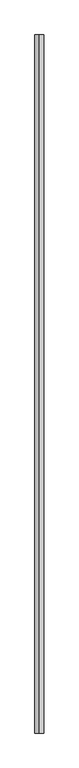
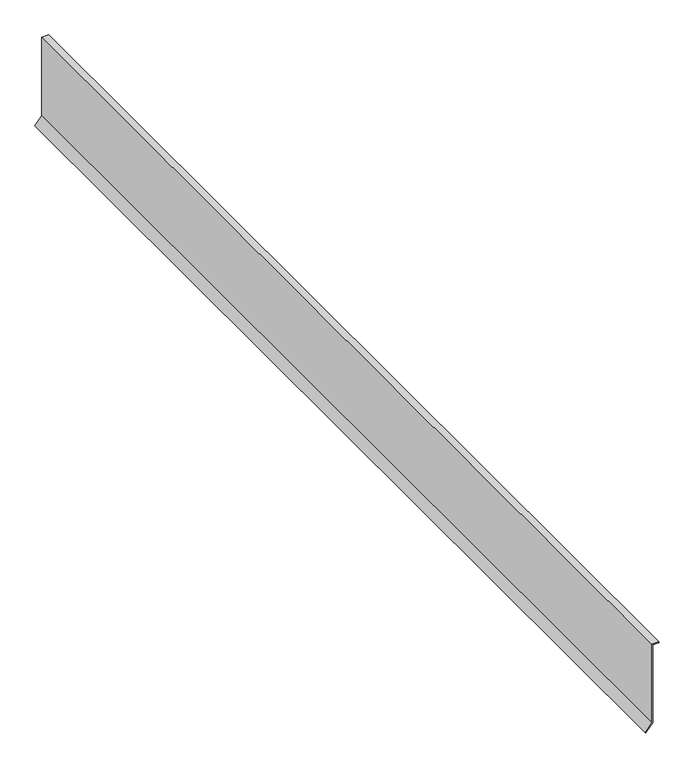
"""IFC4 building model written with IfcOpenShell, lengths in millimetres: proxy geometry, GRAVEL STOP007 14648 : GRAVEL STOP007 14648."""

from ifc_helpers import new_model, si_unit, frame, origin, place, context, project, spatial, polyline, outline, extrude, source, transform, mapped, element, save


def generic_models_a1fe0a36(model_context):
    return source(origin(), model_context, "Body", "SweptSolid", [
        extrude(outline(polyline([(40082.2407116, -2815.6343429), (40081.3605882, -2814.5313394), (40097.4918556, -2801.659661), (40253.3245993, -2801.659661), (40253.3245993, -2789.8917422), (40254.7357103, -2789.8917422), (40254.7357103, -2803.070772), (40097.9858473, -2803.070772), (40082.2407116, -2815.6343429)])), frame((0.0, 999.75, 0.0), z_axis=(0.0, 1.0, 0.0), x_axis=(0.0, 0.0, 1.0)), (0.0, 0.0, 1.0), 2000.25),
    ])


if __name__ == "__main__":
    model = new_model("IFC4")
    model_context = context("Model", 3, world=origin())
    ifc_project = project(units=[si_unit("LENGTHUNIT", "METRE", prefix="MILLI")], contexts=[model_context])
    site = spatial("IfcSite", under=ifc_project)
    building = spatial("IfcBuilding", under=site)
    placement = place(None, origin())
    generic_models_shape = generic_models_a1fe0a36(model_context)
    element("IfcBuildingElementProxy", 1, Name="GRAVEL STOP007 14648 : GRAVEL STOP007 14648", ObjectType="GRAVEL STOP007 14648 : GRAVEL STOP007 14648", at=placement, inside=building, context=model_context, shape_type="MappedRepresentation", body=[
        mapped(generic_models_shape, transform((0.0, 0.0, 0.0), x_axis=(1.0, 0.0, 0.0), y_axis=(0.0, 1.0, 0.0), z_axis=(0.0, 0.0, 1.0))),
    ])
    save(model, "model.ifc")

# Revit data of these elements
# Type "GRAVEL STOP007 14648 : GRAVEL STOP007 14648"
#   NameOverride = "GRAVEL STOP007"
# Element 1 (IfcBuildingElementProxy, "GRAVEL STOP007 14648 : GRAVEL STOP007 14648")
#   Materials on its faces: "GRAVEL STOP REQUIRED WITH GRAVEL SURFACE SYSTEMS"
# Materials
#   "GRAVEL STOP REQUIRED WITH GRAVEL SURFACE SYSTEMS": class "Unassigned", colour RGB 170 170 127, transparency 0
